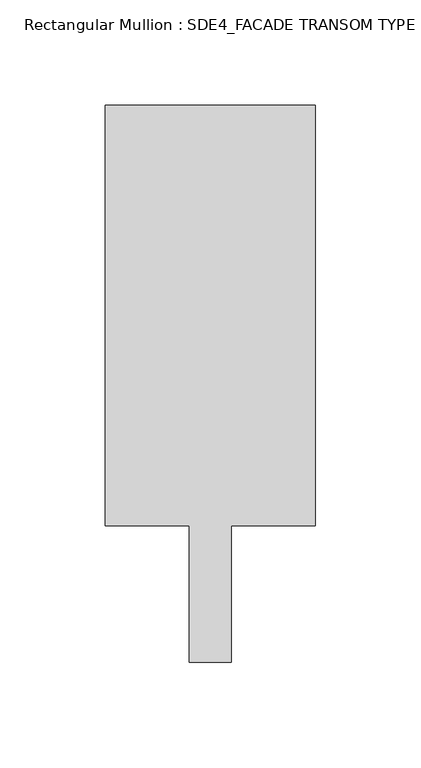
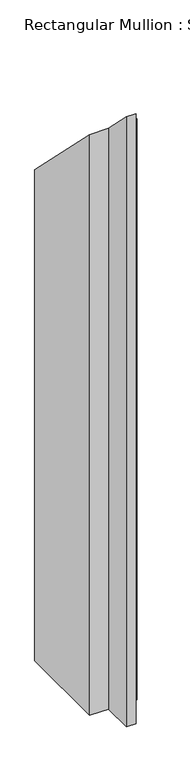
"""IFC4 building model written with IfcOpenShell, lengths in millimetres: member geometry, Rectangular Mullion : SDE4_FACADE TRANSOM TYPE 2."""

from ifc_helpers import new_model, si_unit, origin, place, context, project, spatial, faceted_brep, source, transform, mapped, element, save


def rectangular_mullion_sde4_facade_transom_type_2_b1e3dd36(model_context):
    return source(origin(), model_context, "Body", "Brep", [
        faceted_brep([(50.0, 132.5, -1222.5), (50.0, -67.5, -1222.5), (10.0, -67.5, -1222.5), (10.0, -132.5, -1222.5), (-10.0, -132.5, -1222.5), (-10.0, -67.5, -1222.5), (-50.0, -67.5, -1222.5), (-50.0, 132.5, -1222.5), (-50.0, 132.5, -132.5), (50.0, 132.5, -132.5), (-50.0, -67.5, 67.5), (-10.0, -67.5, 67.5), (-10.0, -132.5, 132.5), (10.0, -132.5, 132.5), (10.0, -67.5, 67.5), (50.0, -67.5, 67.5)], [[[0, 1, 2, 3, 4, 5, 6, 7]], [[8, 9, 0, 7]], [[10, 8, 7, 6]], [[11, 10, 6, 5]], [[12, 11, 5, 4]], [[13, 12, 4, 3]], [[14, 13, 3, 2]], [[15, 14, 2, 1]], [[9, 15, 1, 0]], [[9, 8, 10, 11, 12, 13, 14, 15]]]),
    ])


if __name__ == "__main__":
    model = new_model("IFC4")
    model_context = context("Model", 3, world=origin())
    ifc_project = project(units=[si_unit("LENGTHUNIT", "METRE", prefix="MILLI")], contexts=[model_context])
    site = spatial("IfcSite", under=ifc_project)
    building = spatial("IfcBuilding", under=site)
    placement = place(None, origin())
    rectangular_mullion_sde4_facade_transom_type_2_shape = rectangular_mullion_sde4_facade_transom_type_2_b1e3dd36(model_context)
    element("IfcMember", 1, ObjectType="Rectangular Mullion : SDE4_FACADE TRANSOM TYPE 2", at=placement, inside=building, context=model_context, shape_type="MappedRepresentation", body=[
        mapped(rectangular_mullion_sde4_facade_transom_type_2_shape, transform((0.0, 0.0, 0.0), x_axis=(1.0, 0.0, 0.0), y_axis=(0.0, 1.0, 0.0), z_axis=(0.0, 0.0, 1.0))),
    ])
    save(model, "model.ifc")

# Revit data of these elements
# Type "Rectangular Mullion : SDE4_FACADE TRANSOM TYPE 2"
#   built-in parameter 1007322 = 0.869423 (stored number, unit not read)
#   built-in parameter 1007321 = 0.164042 (stored number, unit not read)
#   built-in parameter 1007320 = 0.164042 (stored number, unit not read)
